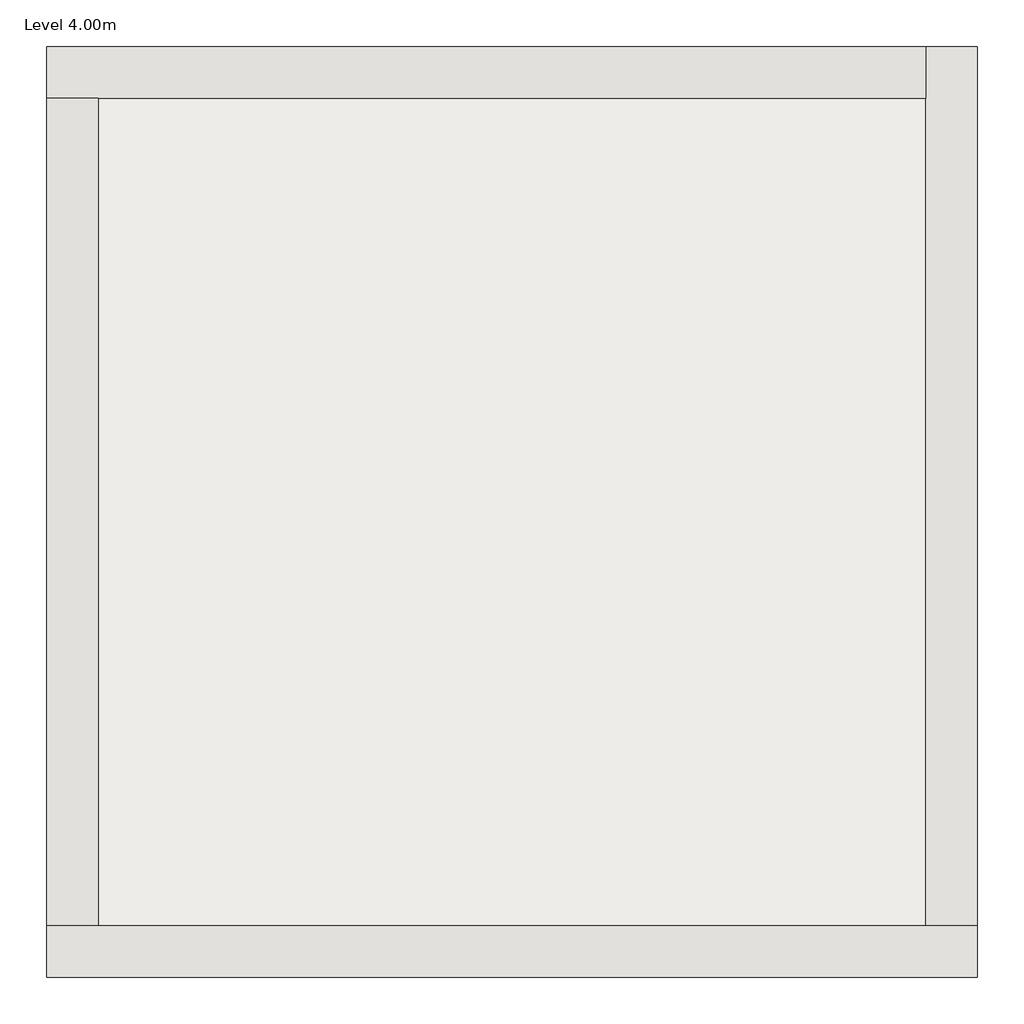
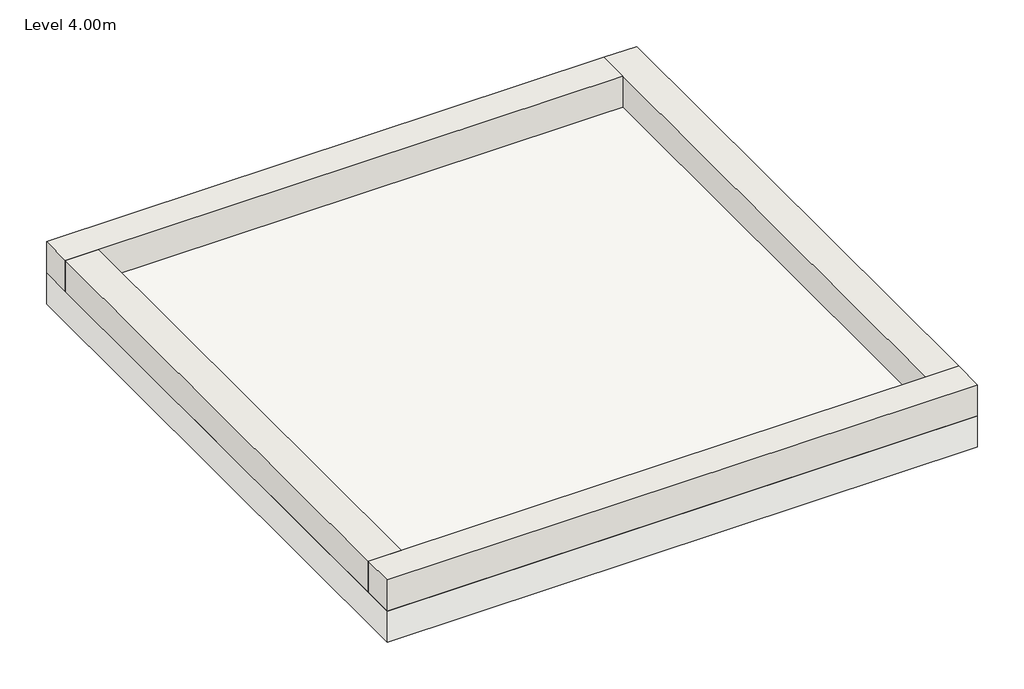
# One storey: 4 walls, 1 slab.
"""IFC4 building model written with IfcOpenShell, lengths in millimetres."""

from ifc_helpers import new_model, si_unit, frame, origin, place, context, project, spatial, polyline, outline, extrude, faceted_brep, element, save

model = new_model("IFC4")

# Units and contexts
model_context = context("Model", 3, world=origin())
ifc_project = project(units=[si_unit("LENGTHUNIT", "METRE", prefix="MILLI")], contexts=[model_context])

# Site, building, storey
site = spatial("IfcSite", under=ifc_project)
building = spatial("IfcBuilding", under=site)
storey = spatial("IfcBuildingStorey", under=building, Name="Level 4.00m", Elevation=4000.0)

# Slab
placement = place(None, origin())
element("IfcSlab", 1, ObjectType="FOR INT AC-NH", at=placement, inside=storey, context=model_context, shape_type="SweptSolid", body=[
    extrude(outline(polyline([(9000.000032, -1000.005872), (0.0, -1000.005872), (0.0, 7999.99416), (9000.000032, 7999.99416), (9000.000032, -1000.005872)])), frame((0.0, 0.0, 3500.0000028), z_axis=(0.0, 0.0, 1.0), x_axis=(1.0, 0.0, 0.0)), (0.0, 0.0, 1.0), 499.9999972),
])

# Walls
element("IfcWall", 2, ObjectType="MURO EXTERIOR0.60", at=placement, inside=storey, context=model_context, shape_type="Brep", body=[
    faceted_brep([(0.0, -1000.005872, 4000.0), (9000.000032, -1000.005872, 4000.0), (9000.000032, -1000.005872, 4499.99392), (0.0, -1000.005872, 4499.99392), (0.0, -500.005856, 4000.0), (0.0, -500.005856, 4499.99392), (500.000016, -500.005856, 4499.99392), (8500.000016, -500.005856, 4499.99392), (9000.000032, -500.005856, 4499.99392), (9000.000032, -500.005856, 4000.0), (8500.000016, -500.005856, 4000.0), (500.000016, -500.005856, 4000.0)], [[[0, 1, 2, 3]], [[4, 5, 6, 7, 8, 9, 10, 11]], [[1, 0, 4, 11, 10, 9]], [[3, 2, 8, 7, 6, 5]], [[2, 1, 9, 8]], [[0, 3, 5, 4]]]),
])
element("IfcWall", 3, ObjectType="MURO EXTERIOR0.60", at=placement, inside=storey, context=model_context, shape_type="Brep", body=[
    faceted_brep([(9000.000032, -500.005856, 4000.0), (9000.000032, 7999.99416, 4000.0), (9000.000032, 7999.99416, 4499.99392), (9000.000032, -500.005856, 4499.99392), (8500.000016, -500.005856, 4000.0), (8500.000016, -500.005856, 4499.99392), (8500.000016, 7499.994144, 4499.99392), (8500.000016, 7999.99416, 4499.99392), (8500.000016, 7999.99416, 4000.0), (8500.000016, 7499.994144, 4000.0)], [[[0, 1, 2, 3]], [[4, 5, 6, 7, 8, 9]], [[1, 0, 4, 9, 8]], [[3, 2, 7, 6, 5]], [[2, 1, 8, 7]], [[0, 3, 5, 4]]]),
])
element("IfcWall", 4, ObjectType="MURO EXTERIOR0.60", at=placement, inside=storey, context=model_context, shape_type="Brep", body=[
    faceted_brep([(8500.000016, 7999.99416, 4000.0), (0.0, 7999.99416, 4000.0), (0.0, 7999.99416, 4499.99392), (8500.000016, 7999.99416, 4499.99392), (8500.000016, 7499.994144, 4000.0), (8500.000016, 7499.994144, 4499.99392), (500.000016, 7499.994144, 4499.99392), (0.0, 7499.994144, 4499.99392), (0.0, 7499.994144, 4000.0), (500.000016, 7499.994144, 4000.0)], [[[0, 1, 2, 3]], [[4, 5, 6, 7, 8, 9]], [[1, 0, 4, 9, 8]], [[3, 2, 7, 6, 5]], [[2, 1, 8, 7]], [[0, 3, 5, 4]]]),
])
element("IfcWall", 5, ObjectType="MURO EXTERIOR0.60", at=placement, inside=storey, context=model_context, shape_type="SweptSolid", body=[
    extrude(outline(polyline([(0.0, -500.005856), (0.0, 7499.994144), (500.000016, 7499.994144), (500.000016, -500.005856), (0.0, -500.005856)])), frame((0.0, 0.0, 4000.0), z_axis=(0.0, 0.0, 1.0), x_axis=(1.0, 0.0, 0.0)), (0.0, 0.0, 1.0), 499.99392),
])

save(model, "model.ifc")

# Revit data of these elements
# Type "FOR INT AC-NH"
#   Layers, outside or top first: 0.010 m "Plaqueta o baldosa de gres" (function 1); 0.055 m "Mortero de cemento o cal para albañilería y para revoco-enlucido d entre 1000 y 1250" (function 1); 0.120 m "Poliestireno Expandido XPS" (function 1); 0.250 m "FU Entrevigado cerámico -Canto 250 mm" (function 1); 0.050 m "Cámara de aire sin ventilar horizontal 5 cm" (function 1); 0.015 m "Placa de yeso laminado (PYL) d entre 750 y 900" (function 1)
# Type "MURO EXTERIOR0.60"
#   Description = "Metal Studs with Brick over sheathing on exterior and Gypsum Wall Board (GWB) on interior, Exterior Function"
#   Assembly Code = "B2010158"
#   Type Mark = "W10"
#   Layers, outside or top first: 0.030 m no material (function 1); 0.140 m no material (function 1); 0.240 m no material (function 1); 0.010 m no material (function 1); 0.050 m no material (function 1); 0.015 m no material (function 1); 0.015 m no material (function 1)
# Element 1 (IfcSlab, "FOR INT AC-NH")
#   Height Offset From Level = 0.000 m
#   Phase Created = New Construction
#   Materials on its faces: "Placa de yeso laminado (PYL) d entre 750 y 900", "Plaqueta o baldosa de gres"
# Elements 2, 3, 4, 5 (IfcWall, "MURO EXTERIOR0.60")
#   Top Offset = 0.000 m
#   Base Offset = 0.000 m
#   Unconnected Height = 0.499994 m
#   wall height = 0.499994 m
#   Phase Created = New Construction
#   Base Constraint = Level 4.00m
#   Materials on its faces: "Default Wall"
# Materials
#   "Plaqueta o baldosa de gres": class "Cerámicos", colour RGB 0 0 0, transparency 0, Comments = "CTE"
#   "Mortero de cemento o cal para albañilería y para revoco-enlucido d entre 1000 y 1250": class "Morteros", colour RGB 0 0 0, transparency 0, Comments = "CTE"
#   "Poliestireno Expandido XPS": class "Plásticos", colour RGB 0 0 0, transparency 0, Comments = "CTE"
#   "FU Entrevigado cerámico -Canto 250 mm": class "Forjados unidireccionales", colour RGB 0 0 0, transparency 0, Comments = "CTE"
#   "Cámara de aire sin ventilar horizontal 5 cm": class "Cámaras de aire", colour RGB 0 0 0, transparency 0, Comments = "CTE"
#   "Placa de yeso laminado (PYL) d entre 750 y 900": class "Yesos", colour RGB 0 0 0, transparency 0, Comments = "CTE"
#   "Default Wall": class "Miscellaneous", colour RGB 192 192 192, transparency 0, Cost = 0
